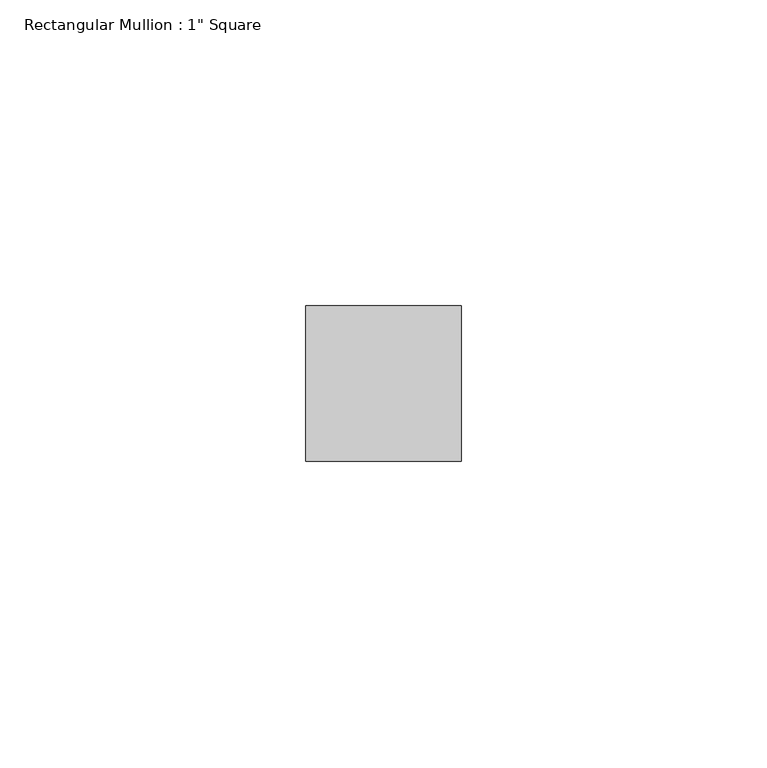
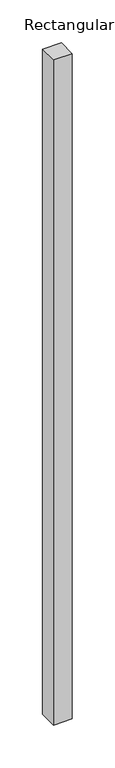
"""IFC4 building model written with IfcOpenShell, lengths in millimetres: member geometry."""

from ifc_helpers import new_model, si_unit, frame, origin, place, context, project, spatial, polyline, outline, extrude, source, transform, mapped, element, save


def member_5bd2dbfd(model_context):
    return source(origin(), model_context, "Body", "SweptSolid", [
        extrude(outline(polyline([(0.0, 12.7), (0.0, -12.7), (-25.4, -12.7), (-25.4, 12.7), (0.0, 12.7)])), frame((0.0, 0.0, -949.4191728), z_axis=(0.0, 0.0, 1.0), x_axis=(1.0, 0.0, 0.0)), (0.0, 0.0, 1.0), 949.4191728),
    ])


if __name__ == "__main__":
    model = new_model("IFC4")
    model_context = context("Model", 3, world=origin())
    ifc_project = project(units=[si_unit("LENGTHUNIT", "METRE", prefix="MILLI")], contexts=[model_context])
    site = spatial("IfcSite", under=ifc_project)
    building = spatial("IfcBuilding", under=site)
    placement = place(None, origin())
    member_shape = member_5bd2dbfd(model_context)
    element("IfcMember", 1, ObjectType="Rectangular Mullion : 1\" Square", at=placement, inside=building, context=model_context, shape_type="MappedRepresentation", body=[
        mapped(member_shape, transform((0.0, 0.0, 0.0), x_axis=(1.0, 0.0, 0.0), y_axis=(0.0, 1.0, 0.0), z_axis=(0.0, 0.0, 1.0))),
    ])
    save(model, "model.ifc")

# Revit data of these elements
# Type "Rectangular Mullion : 1\" Square"
#   built-in parameter 1007304 = 0.0833333 (stored number, unit not read)
#   built-in parameter 1007301 = 0.0416667 (stored number, unit not read)
#   built-in parameter 1007300 = 0.0416667 (stored number, unit not read)
# Element 1 (IfcMember, "Rectangular Mullion : 1\" Square")
#   Materials on its faces: "Metal - Aluminum"
# Materials
#   "Metal - Aluminum": class "Metal", colour RGB 247 247 247, transparency 0
